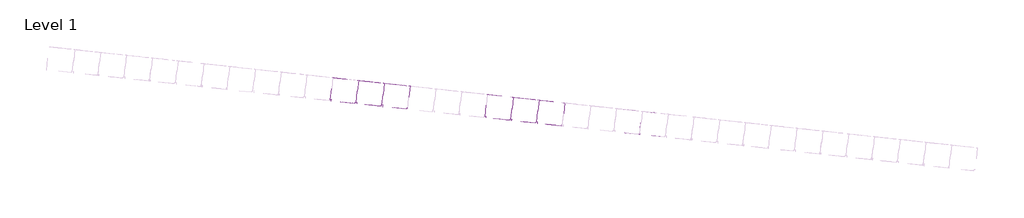
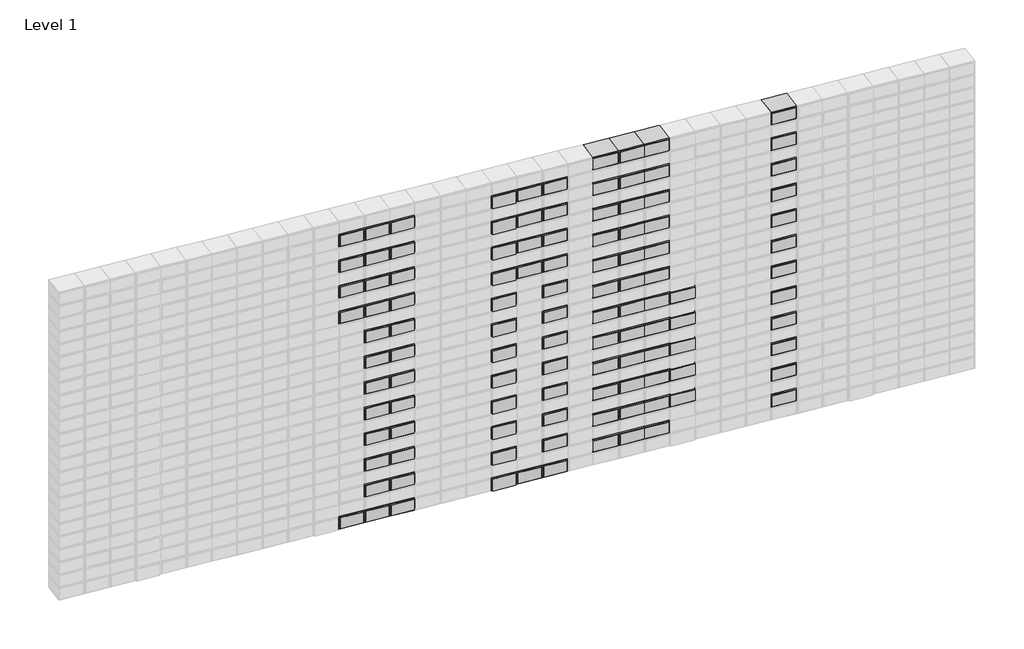
# One storey, part 15 of 18: 111 proxies.
# Revit data of these elements (continued)
# Elements 37, 38, 39, 40, 41, 42, 43, 44, 45, 46, 47, 48, 49, 50, 51, 52, 53 (IfcBuildingElementProxy, "00_GMA_steen_versie_6 : Geel") (continued)
#   Materials on its faces: "20_voeg", "21_steen_geel"
# Elements 54, 55, 56, 57, 58, 59, 60, 61, 62, 63, 64, 65, 66, 67, 68, 69, 70, 71, 72, 73, 74, 75, 76, 77, 78, 79, 80, 81, 82, 83, 84, 85, 86, 87, 88, 89, 90, 91, 92, 93, 94, 95, 96, 97, 98, 99 (IfcBuildingElementProxy, "00_GMA_steen_versie_6 : Rood")
#   StootvoegLinksHalfOnder = 5 mm
#   StootvoegLinksHalfBoven = 5 mm
#   StootVoegRechtsHalfOnder = 5 mm
#   StootVoegRechtsHalfBoven = 5 mm
#   StootVoegBreedteRechts = 10 mm
#   StootVoegBreedteLinks = 10 mm
#   LintVoegOnderHalf = 5 mm
#   LintVoegOnder = 10 mm
#   LintVoegBovenHalf = 5 mm
#   LintVoegBoven = 10 mm
#   Phase Created = New Construction
#   Materials on its faces: "20_voeg", "21_steen_rood"
# Elements 100, 101, 102, 103, 104, 105, 106, 107, 108, 109, 110, 111 (IfcBuildingElementProxy, "00_GMA_steen_versie_6 : Rood")
#   StootvoegLinksHalfOnder = 5 mm
#   StootvoegLinksHalfBoven = 5 mm
#   StootVoegRechtsHalfOnder = 5 mm
#   StootVoegRechtsHalfBoven = 5 mm
#   StootVoegBreedteRechts = 10 mm
#   StootVoegBreedteLinks = 10 mm
#   LintVoegOnderHalf = 0 mm
#   LintVoegOnder = 0 mm
#   LintVoegBovenHalf = 5 mm
#   LintVoegBoven = 10 mm
#   Phase Created = New Construction
#   Materials on its faces: "20_voeg", "21_steen_rood"
# Materials
#   "21_steen_geel": class "Unassigned", colour RGB 202 202 0, transparency 0, Cost = 0
#   "20_voeg": class "Concrete", colour RGB 86 86 86, transparency 0, Manufacturer = "RevitGG", URL = "www.revitgg.nl", Description = "zandcement, generiek materiaal", Cost = 0
#   "21_steen_rood": class "Unassigned", colour RGB 213 111 43, transparency 0, Cost = 0
